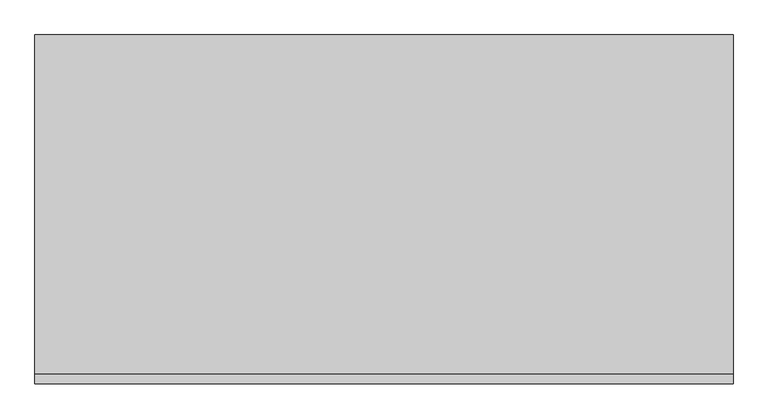
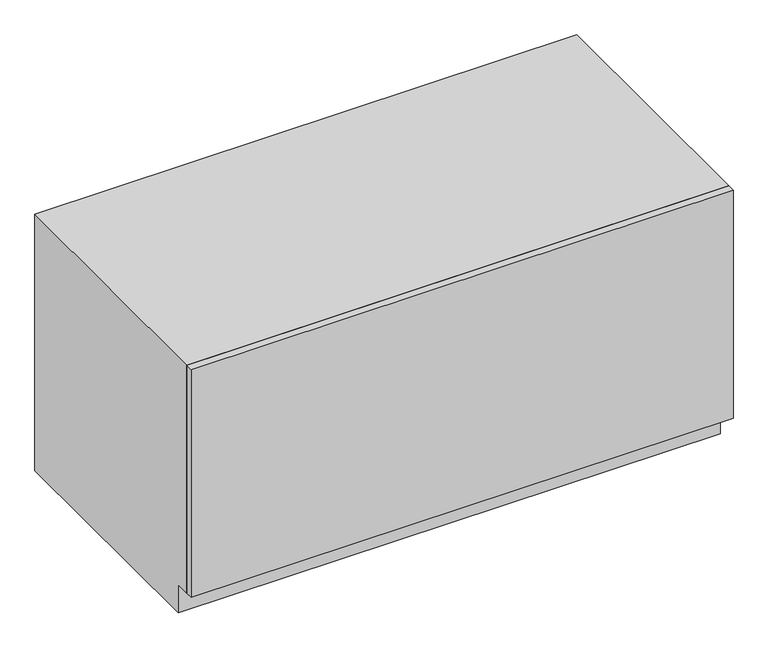
"""IFC4 building model written with IfcOpenShell, lengths in millimetres: furniture geometry, OD_CW_Base Cabinet : OD_CW_Base Cabinet."""

import ifcopenshell
import ifcopenshell.guid

model = None  # the IFC model being written
_history = None  # IfcOwnerHistory: only IFC2X3 demands one
_inside = {}  # id of a spatial element -> (the spatial element, [elements in it])
_under = {}  # id of a project, library or spatial element -> (it, [spatial elements below it])
_declared = {}  # id of a project -> (the project, [libraries it declares])
_typed = {}  # id of a type object -> (the type object, [elements of that type])
_made_of = {}  # id of a material, layer set ... -> (it, [elements and type objects made of it])


def new_model(schema):
    """Start an empty IFC model of exactly this schema.

    Asked for "IFC4X3", IfcOpenShell would pick the latest addendum, in which some entities
    have other attributes; the version numbers below select the first issue.
    IFC2X3 requires an IfcOwnerHistory on every rooted entity: one is made here for all.
    """
    global model, _history
    if schema == "IFC4X3":
        model = ifcopenshell.file(schema_version=(4, 3, 0, 0))
    else:
        model = ifcopenshell.file(schema=schema)
    _inside.clear()
    _under.clear()
    _declared.clear()
    _typed.clear()
    _made_of.clear()
    _history = None
    if model.schema == "IFC2X3":
        org = make("IfcOrganization", Name="unknown")
        user = make(
            "IfcPersonAndOrganization",
            ThePerson=make("IfcPerson", FamilyName="unknown"),
            TheOrganization=org,
        )
        app = make(
            "IfcApplication",
            ApplicationDeveloper=org,
            Version="unknown",
            ApplicationFullName="unknown",
            ApplicationIdentifier="unknown",
        )
        _history = make(
            "IfcOwnerHistory",
            OwningUser=user,
            OwningApplication=app,
            ChangeAction="ADDED",
            CreationDate=0,
        )
    return model


def make(cls, **values):
    """One entity of the class cls with the attributes given. An attribute that is None is left unset."""
    return model.create_entity(
        cls, **{name: value for name, value in values.items() if value is not None}
    )


def rooted(cls, **values):
    """An entity with a GlobalId (a new one), such as an element, a storey or a relation."""
    return make(cls, GlobalId=ifcopenshell.guid.new(), OwnerHistory=_history, **values)


def si_unit(unit_type, name, prefix=None):
    """IfcSIUnit, for example si_unit("LENGTHUNIT", "METRE", prefix="MILLI")."""
    return make("IfcSIUnit", UnitType=unit_type, Prefix=prefix, Name=name)


def assignment(units):
    """IfcUnitAssignment: the units of a project."""
    return None if units is None else make("IfcUnitAssignment", Units=units)


def point(xyz):
    """IfcCartesianPoint."""
    return None if xyz is None else make("IfcCartesianPoint", Coordinates=xyz)


def direction(xyz):
    """IfcDirection."""
    return None if xyz is None else make("IfcDirection", DirectionRatios=xyz)


def frame(location, z_axis=None, x_axis=None):
    """IfcAxis2Placement3D, a coordinate frame: its origin and axes. An axis left out is left unset."""
    return make(
        "IfcAxis2Placement3D",
        Location=point(location),
        Axis=direction(z_axis),
        RefDirection=direction(x_axis),
    )


def origin():
    """The frame at (0, 0, 0) with its axes left unset."""
    return frame((0.0, 0.0, 0.0))


def place(relative_to, where):
    """IfcLocalPlacement: puts the frame where relative to a parent placement (None: the world)."""
    return make(
        "IfcLocalPlacement", PlacementRelTo=relative_to, RelativePlacement=where
    )


def context(
    kind, dimensions, precision=None, world=None, true_north=None, identifier=None
):
    """IfcGeometricRepresentationContext, for example the 3D "Model" context."""
    return make(
        "IfcGeometricRepresentationContext",
        ContextIdentifier=identifier,
        ContextType=kind,
        CoordinateSpaceDimension=dimensions,
        Precision=precision,
        WorldCoordinateSystem=world,
        TrueNorth=true_north,
    )


def project(units=None, contexts=None):
    """IfcProject with its units and contexts."""
    return rooted(
        "IfcProject",
        Name="project",
        RepresentationContexts=contexts,
        UnitsInContext=assignment(units),
    )


def spatial(cls, under=None, at=None, **own):
    """A site, building, storey or space (cls), placed at a placement, below another one or the project."""
    s = rooted(cls, ObjectPlacement=at, **own)
    if under is not None:
        _under.setdefault(under.id(), (under, []))[1].append(s)
    return s


def polyline(points):
    """IfcPolyline through the points."""
    return make("IfcPolyline", Points=[point(p) for p in points])


def outline(outer, holes=None, kind="AREA"):
    """IfcArbitraryClosedProfileDef: a profile drawn as a closed curve; with holes, ...WithVoids."""
    if holes is None:
        return make("IfcArbitraryClosedProfileDef", ProfileType=kind, OuterCurve=outer)
    return make(
        "IfcArbitraryProfileDefWithVoids",
        ProfileType=kind,
        OuterCurve=outer,
        InnerCurves=holes,
    )


def extrude(swept, where, along, depth):
    """IfcExtrudedAreaSolid: the profile swept, set in the frame where, extruded along a direction by depth."""
    return make(
        "IfcExtrudedAreaSolid",
        SweptArea=swept,
        Position=where,
        ExtrudedDirection=direction(along),
        Depth=depth,
    )


def shape(context_of_items, identifier, shape_type, items):
    """IfcShapeRepresentation: the items that make up one representation, for example the "Body"."""
    return make(
        "IfcShapeRepresentation",
        ContextOfItems=context_of_items,
        RepresentationIdentifier=identifier,
        RepresentationType=shape_type,
        Items=items,
    )


def source(mapping_origin, context_of_items, identifier, shape_type, items):
    """IfcRepresentationMap: a shape defined once, which mapped items show again and again."""
    return make(
        "IfcRepresentationMap",
        MappingOrigin=mapping_origin,
        MappedRepresentation=shape(context_of_items, identifier, shape_type, items),
    )


def transform(
    local_origin,
    x_axis=None,
    y_axis=None,
    z_axis=None,
    scale=None,
    scale2=None,
    scale3=None,
    uniform=True,
):
    """IfcCartesianTransformationOperator3D, or its non-uniform kind. x_axis, y_axis, z_axis: its Axis1, 2, 3."""
    if uniform:
        return make(
            "IfcCartesianTransformationOperator3D",
            Axis1=direction(x_axis),
            Axis2=direction(y_axis),
            LocalOrigin=point(local_origin),
            Scale=scale,
            Axis3=direction(z_axis),
        )
    return make(
        "IfcCartesianTransformationOperator3DnonUniform",
        Axis1=direction(x_axis),
        Axis2=direction(y_axis),
        LocalOrigin=point(local_origin),
        Scale=scale,
        Axis3=direction(z_axis),
        Scale2=scale2,
        Scale3=scale3,
    )


def mapped(mapping_source, mapping_target):
    """IfcMappedItem: shows the shape of a source again, moved by a transform."""
    return make(
        "IfcMappedItem", MappingSource=mapping_source, MappingTarget=mapping_target
    )


def made_of(thing, what):
    """Note that an element or type object is made of a material, layer set ...; save() writes the relation."""
    if what is not None:
        _made_of.setdefault(what.id(), (what, []))[1].append(thing)
    return thing


def element(
    cls,
    number,
    at=None,
    inside=None,
    cuts=None,
    type_object=None,
    material=None,
    context=None,
    identifier="Body",
    shape_type=None,
    held_by="IfcProductDefinitionShape",
    body=None,
    shapes=None,
    **own,
):
    """One element of the class cls, such as IfcWall. Its Tag is "e" and its number.

    at: its placement. inside: the storey or other place that contains it. cuts: it is an
    opening in that element (IfcRelVoidsElement). A single representation is given by context,
    identifier, shape_type and body (its items); several are given by shapes. held_by: the class
    of the entity that holds the representations. save() writes the other relations.
    """
    e = rooted(cls, Tag="e%d" % number, ObjectPlacement=at, **own)
    if body is not None:
        shapes = [shape(context, identifier, shape_type, body)]
    if shapes is not None:
        e.Representation = make(held_by, Representations=shapes)
    if inside is not None:
        _inside.setdefault(inside.id(), (inside, []))[1].append(e)
    if cuts is not None:
        rooted(
            "IfcRelVoidsElement", RelatingBuildingElement=cuts, RelatedOpeningElement=e
        )
    if type_object is not None:
        _typed.setdefault(type_object.id(), (type_object, []))[1].append(e)
    return made_of(e, material)


def aggregate(whole, parts):
    """IfcRelAggregates: a whole, such as a stair, and the parts it consists of."""
    return rooted("IfcRelAggregates", RelatingObject=whole, RelatedObjects=parts)


def save(model, path):
    """Write the relations noted so far, then the file.

    IfcRelAggregates (storeys below a building ...), IfcRelContainedInSpatialStructure (elements
    in a storey), IfcRelDefinesByType, IfcRelAssociatesMaterial and IfcRelDeclares: one each for
    every whole, place, type object, material and project.
    """
    for whole, parts in _under.values():
        aggregate(whole, parts)
    for where, things in _inside.values():
        rooted(
            "IfcRelContainedInSpatialStructure",
            RelatedElements=things,
            RelatingStructure=where,
        )
    for kind, things in _typed.values():
        rooted("IfcRelDefinesByType", RelatedObjects=things, RelatingType=kind)
    for what, things in _made_of.values():
        rooted("IfcRelAssociatesMaterial", RelatedObjects=things, RelatingMaterial=what)
    for by, libraries in _declared.values():
        rooted("IfcRelDeclares", RelatingContext=by, RelatedDefinitions=libraries)
    model.write(path)


def furniture_1602f4be(model_context):
    return source(origin(), model_context, "Body", "SweptSolid", [
        extrude(outline(polyline([(18.7377049, -279.4), (1847.5377049, -279.4), (1847.5377049, -304.8), (18.7377049, -304.8), (18.7377049, -279.4)])), frame((0.0, 0.0, 101.6), z_axis=(0.0, 0.0, 1.0), x_axis=(1.0, 0.0, 0.0)), (0.0, 0.0, 1.0), 812.8),
        extrude(outline(polyline([(-279.4, 914.4), (609.6, 914.4), (609.6, 0.0), (-228.6, 0.0), (-228.6, 101.6), (-279.4, 101.6), (-279.4, 914.4)])), frame((18.7377049, 0.0, 0.0), z_axis=(1.0, 0.0, 0.0), x_axis=(0.0, 1.0, 0.0)), (0.0, 0.0, 1.0), 1828.8),
    ])


if __name__ == "__main__":
    model = new_model("IFC4")
    model_context = context("Model", 3, world=origin())
    ifc_project = project(units=[si_unit("LENGTHUNIT", "METRE", prefix="MILLI")], contexts=[model_context])
    site = spatial("IfcSite", under=ifc_project)
    building = spatial("IfcBuilding", under=site)
    placement = place(None, origin())
    furniture_shape = furniture_1602f4be(model_context)
    element("IfcFurniture", 1, ObjectType="OD_CW_Base Cabinet : OD_CW_Base Cabinet", at=placement, inside=building, context=model_context, shape_type="MappedRepresentation", body=[
        mapped(furniture_shape, transform((0.0, 0.0, 0.0), x_axis=(1.0, 0.0, 0.0), y_axis=(0.0, 1.0, 0.0), z_axis=(0.0, 0.0, 1.0))),
    ])
    save(model, "model.ifc")

# Revit data of these elements
# Type "OD_CW_Base Cabinet : OD_CW_Base Cabinet"
#   OD_CW_Width [instance default] = 2' - 10"
#   OD_CW_Length [instance default] = 8' - 0"
#   OD_CW_Height [instance default] = 2' - 3"
#   Depth = 2' - 0"
#   Height = 3' - 0"
#   Width = 4' - 0"
#   OD_CW_Material_Front Panel [instance default] = none
#   OD_CW_Material_Body [instance default] = none
# Element 1 (IfcFurniture, "OD_CW_Base Cabinet : OD_CW_Base Cabinet")
#   OD_CW_Width = 3' - 0"
#   OD_CW_Length = 6' - 0"
#   OD_CW_Height = 3' - 0"
#   OD_CW_Material_Body = SALAD COOLER
#   Materials on its faces: "SALAD COOLER", "CASEWORK"
# Materials
#   "SALAD COOLER": class "Generic", colour RGB 187 187 187, transparency 0, Cost = 0
#   "CASEWORK": class "Generic", colour RGB 181 181 181, transparency 0, Cost = 0
